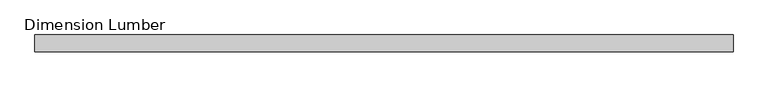
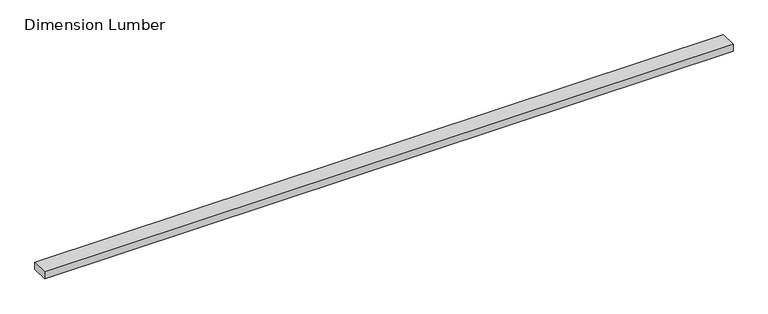
"""IFC4 building model written with IfcOpenShell, lengths in millimetres: beam geometry, Dimension Lumber : Top Supporting Lumbers."""

from ifc_helpers import new_model, si_unit, frame, origin, place, context, project, spatial, polyline, outline, extrude, source, transform, mapped, element, save


def dimension_lumber_ec547c4e(model_context):
    return source(origin(), model_context, "Body", "SweptSolid", [
        extrude(outline(polyline([(1866.9, 44.45), (1866.9, -44.45), (-1809.75, -44.45), (-1809.75, 44.45), (1866.9, 44.45)])), frame((0.0, 0.0, -19.05), z_axis=(0.0, 0.0, 1.0), x_axis=(1.0, 0.0, 0.0)), (0.0, 0.0, 1.0), 38.1),
    ])


if __name__ == "__main__":
    model = new_model("IFC4")
    model_context = context("Model", 3, world=origin())
    ifc_project = project(units=[si_unit("LENGTHUNIT", "METRE", prefix="MILLI")], contexts=[model_context])
    site = spatial("IfcSite", under=ifc_project)
    building = spatial("IfcBuilding", under=site)
    placement = place(None, origin())
    dimension_lumber_shape = dimension_lumber_ec547c4e(model_context)
    element("IfcBeam", 1, ObjectType="Dimension Lumber : Top Supporting Lumbers", at=placement, inside=building, context=model_context, shape_type="MappedRepresentation", body=[
        mapped(dimension_lumber_shape, transform((0.0, 0.0, 0.0), x_axis=(1.0, 0.0, 0.0), y_axis=(0.0, 1.0, 0.0), z_axis=(0.0, 0.0, 1.0))),
    ])
    save(model, "model.ifc")

# Revit data of these elements
# Type "Dimension Lumber : Top Supporting Lumbers"
#   Assembly Code = "B10"
#   A = 0.0364583 SF
#   Length [instance default] = 5' - 0"
#   b = 0' - 3 1/2"
#   d = 0' - 1 1/2"
#   Structural Material [instance default] = Softwood, Lumber
# Element 1 (IfcBeam, "Dimension Lumber : Top Supporting Lumbers")
#   Structural Material = Douglas Fir #2
#   Materials on its faces: "Douglas Fir #2"
# Materials
#   "Softwood, Lumber": class "Wood", colour RGB 223 192 134, transparency 0, Description = "Pinus Echinata", Cost = 0
#   "Douglas Fir #2": class "Wood", colour RGB 223 192 134, transparency 0, Description = "Pinus Echinata", Cost = 0
